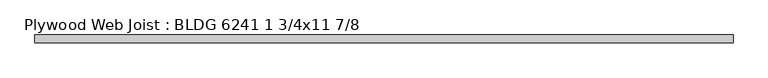
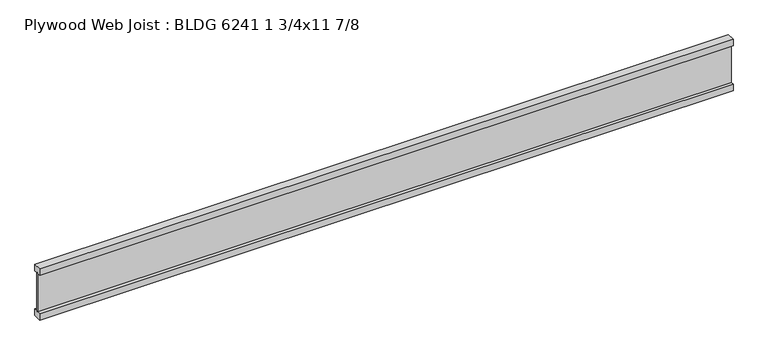
"""IFC4 building model written with IfcOpenShell, lengths in millimetres: beam geometry, Plywood Web Joist : BLDG 6241 1 3/4x11 7/8."""

from ifc_helpers import new_model, si_unit, frame, origin, place, context, project, spatial, polyline, outline, extrude, source, transform, mapped, element, save


def plywood_web_joist_bldg_6241_1_3_4x11_7_8_9cf04d55(model_context):
    return source(origin(), model_context, "Body", "SweptSolid", [
        extrude(outline(polyline([(-22.225, 150.8125), (22.225, 150.8125), (22.225, 112.7125), (4.7625, 112.7125), (4.7625, 119.0625), (-4.7625, 119.0625), (-4.7625, 112.7125), (-22.225, 112.7125), (-22.225, 150.8125)])), frame((-1927.225, 0.0, 0.0), z_axis=(1.0, 0.0, 0.0), x_axis=(0.0, 1.0, 0.0)), (0.0, 0.0, 1.0), 3854.45),
        extrude(outline(polyline([(22.225, -112.7125), (22.225, -150.8125), (-22.225, -150.8125), (-22.225, -112.7125), (-4.7625, -112.7125), (-4.7625, -118.3285374), (4.7625, -118.3285374), (4.7625, -112.7125), (22.225, -112.7125)])), frame((-1927.225, 0.0, 0.0), z_axis=(1.0, 0.0, 0.0), x_axis=(0.0, 1.0, 0.0)), (0.0, 0.0, 1.0), 3854.45),
        extrude(outline(polyline([(1927.225, 4.7625), (1927.225, -4.7625), (-1927.225, -4.7625), (-1927.225, 4.7625), (1927.225, 4.7625)])), frame((0.0, 0.0, -118.3285374), z_axis=(0.0, 0.0, 1.0), x_axis=(1.0, 0.0, 0.0)), (0.0, 0.0, 1.0), 237.3910374),
    ])


if __name__ == "__main__":
    model = new_model("IFC4")
    model_context = context("Model", 3, world=origin())
    ifc_project = project(units=[si_unit("LENGTHUNIT", "METRE", prefix="MILLI")], contexts=[model_context])
    site = spatial("IfcSite", under=ifc_project)
    building = spatial("IfcBuilding", under=site)
    placement = place(None, origin())
    plywood_web_joist_bldg_6241_1_3_4x11_7_8_shape = plywood_web_joist_bldg_6241_1_3_4x11_7_8_9cf04d55(model_context)
    element("IfcBeam", 1, ObjectType="Plywood Web Joist : BLDG 6241 1 3/4x11 7/8", at=placement, inside=building, context=model_context, shape_type="MappedRepresentation", body=[
        mapped(plywood_web_joist_bldg_6241_1_3_4x11_7_8_shape, transform((0.0, 0.0, 0.0), x_axis=(1.0, 0.0, 0.0), y_axis=(0.0, 1.0, 0.0), z_axis=(0.0, 0.0, 1.0))),
    ])
    save(model, "model.ifc")

# Revit data of these elements
# Type "Plywood Web Joist : BLDG 6241 1 3/4x11 7/8"
#   Assembly Code = "B10"
#   Length [instance default] = 5' - 0"
#   b = 0' - 1 3/4"
#   d = 0' - 11 7/8"
#   Structural Material [instance default] = Softwood, Lumber
# Element 1 (IfcBeam, "Plywood Web Joist : BLDG 6241 1 3/4x11 7/8")
#   Materials on its faces: "Softwood, Lumber"
# Materials
#   "Softwood, Lumber": class "Wood", colour RGB 223 192 134, transparency 0, Description = "Pinus Echinata", Cost = 0
